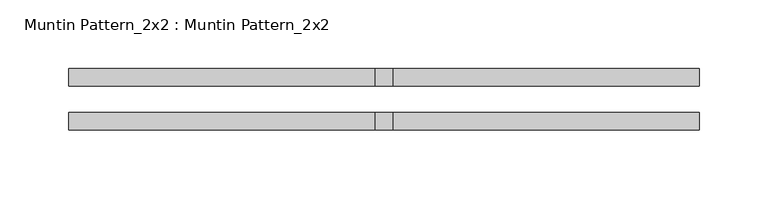
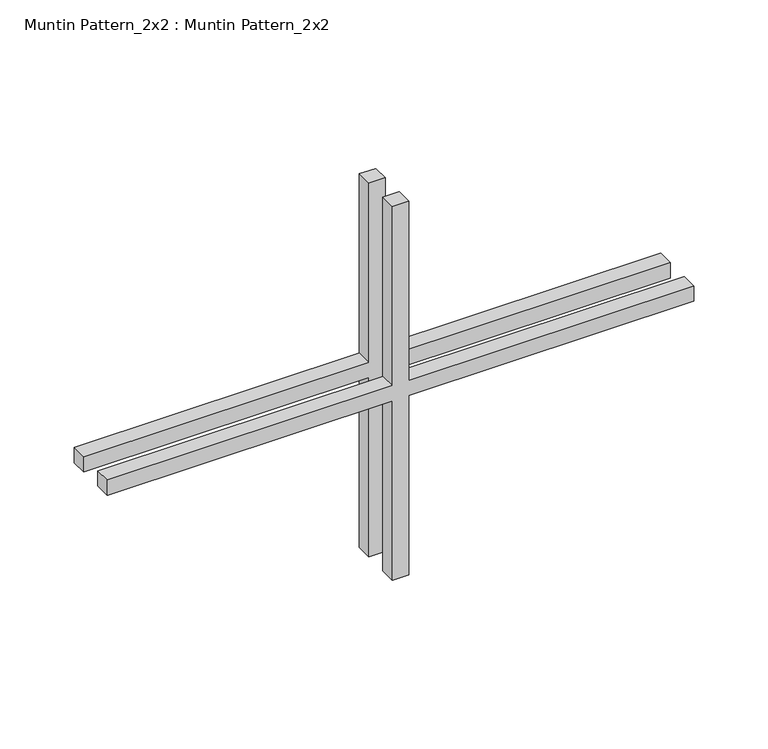
"""IFC4 building model written with IfcOpenShell, lengths in millimetres: proxy geometry, Muntin Pattern_2x2 : Muntin Pattern_2x2."""

from ifc_helpers import new_model, si_unit, frame, origin, place, context, project, spatial, polyline, outline, extrude, source, transform, mapped, element, save


def muntin_pattern_2x2_muntin_pattern_2x2_9e1d4840(model_context):
    return source(origin(), model_context, "Body", "SweptSolid", [
        extrude(outline(polyline([(160.3375, -6.35), (160.3375, -228.6), (147.6375, -228.6), (147.6375, -6.35), (0.0, -6.35), (0.0, 6.35), (147.6375, 6.35), (147.6375, 228.6), (160.3375, 228.6), (160.3375, 6.35), (307.975, 6.35), (307.975, -6.35), (160.3375, -6.35)])), frame((0.0, 9.525, 0.0), z_axis=(0.0, 1.0, 0.0), x_axis=(0.0, 0.0, 1.0)), (0.0, 0.0, 1.0), 12.7),
        extrude(outline(polyline([(160.3375, -6.35), (160.3375, -228.6), (147.6375, -228.6), (147.6375, -6.35), (0.0, -6.35), (0.0, 6.35), (147.6375, 6.35), (147.6375, 228.6), (160.3375, 228.6), (160.3375, 6.35), (307.975, 6.35), (307.975, -6.35), (160.3375, -6.35)])), frame((0.0, -22.225, 0.0), z_axis=(0.0, 1.0, 0.0), x_axis=(0.0, 0.0, 1.0)), (0.0, 0.0, 1.0), 12.7),
    ])


if __name__ == "__main__":
    model = new_model("IFC4")
    model_context = context("Model", 3, world=origin())
    ifc_project = project(units=[si_unit("LENGTHUNIT", "METRE", prefix="MILLI")], contexts=[model_context])
    site = spatial("IfcSite", under=ifc_project)
    building = spatial("IfcBuilding", under=site)
    placement = place(None, origin())
    muntin_pattern_2x2_muntin_pattern_2x2_shape = muntin_pattern_2x2_muntin_pattern_2x2_9e1d4840(model_context)
    element("IfcBuildingElementProxy", 1, Name="Muntin Pattern_2x2 : Muntin Pattern_2x2", ObjectType="Muntin Pattern_2x2 : Muntin Pattern_2x2", at=placement, inside=building, context=model_context, shape_type="MappedRepresentation", body=[
        mapped(muntin_pattern_2x2_muntin_pattern_2x2_shape, transform((0.0, 0.0, 0.0), x_axis=(1.0, 0.0, 0.0), y_axis=(0.0, 1.0, 0.0), z_axis=(0.0, 0.0, 1.0))),
    ])
    save(model, "model.ifc")

# Revit data of these elements
# Type "Muntin Pattern_2x2 : Muntin Pattern_2x2"
#   Width [instance default] = 4' - 0"
#   Thickness = 0' - 0 1/2"
#   Height [instance default] = 4' - 0"
#   Distance = 0' - 0 3/4"
#   Interior Material [instance default] = none
#   Exterior Material [instance default] = none
#   Default Elevation = 0
# Element 1 (IfcBuildingElementProxy, "Muntin Pattern_2x2 : Muntin Pattern_2x2")
#   Width = 1' - 6"
#   Height = 1' - 0 1/8"
#   Interior Material = Wood - Stained
#   Exterior Material = Clad - White
#   Materials on its faces: "Clad - White", "Wood - Stained"
# Materials
#   "Clad - White": class "Wood", colour RGB 242 242 238, transparency 0, Cost = 0
#   "Wood - Stained": class "Wood", colour RGB 224 178 126, transparency 0, Cost = 0
